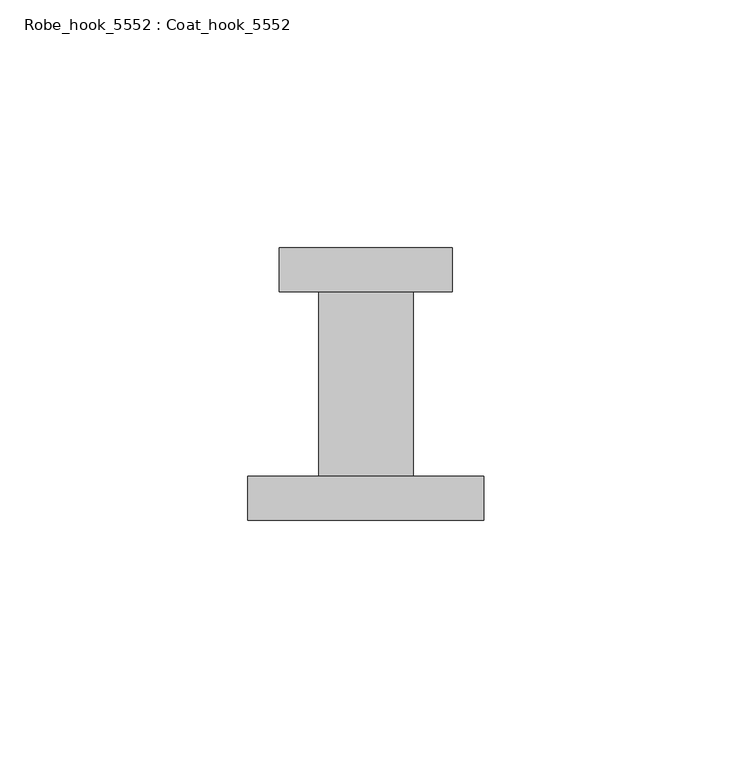
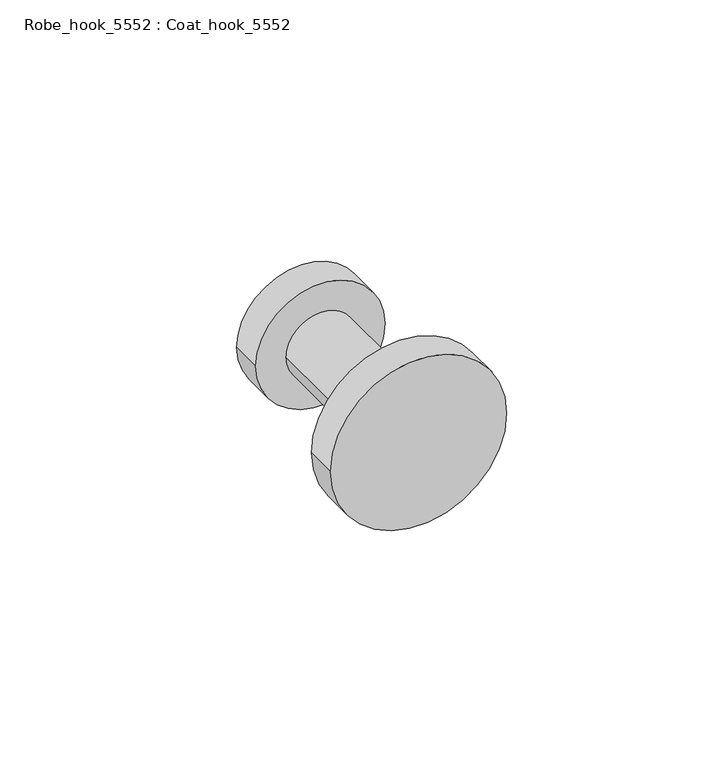
"""IFC4 building model written with IfcOpenShell, lengths in millimetres: proxy geometry, Robe_hook_5552 : Coat_hook_5552."""

from ifc_helpers import new_model, si_unit, point, frame, frame_2d, origin, place, context, project, spatial, circle_curve, trimmed, segment, composite_curve, outline, extrude, source, transform, mapped, element, save


def robe_hook_5552_coat_hook_5552_50ae73f2(model_context):
    return source(origin(), model_context, "Body", "SweptSolid", [
        extrude(outline(composite_curve([segment(trimmed(circle_curve(frame_2d((1371.6, 0.0)), 17.4626016), [point((1371.6, 17.4626016))], [point((1371.6, -17.4626016))], False, "CARTESIAN"), True, "CONTINUOUS"), segment(trimmed(circle_curve(frame_2d((1371.6, 0.0)), 17.4626016), [point((1371.6, -17.4626016))], [point((1371.6, 17.4626016))], False, "CARTESIAN"), True, "CONTINUOUS")], self_intersect=False)), frame((0.0, 46.0399015, 0.0), z_axis=(0.0, 1.0, 0.0), x_axis=(0.0, 0.0, 1.0)), (0.0, 0.0, 1.0), 8.9023917),
        extrude(outline(composite_curve([segment(trimmed(circle_curve(frame_2d((1371.6, 0.0)), 9.525), [point((1371.6, 9.525))], [point((1371.6, -9.525))], False, "CARTESIAN"), True, "CONTINUOUS"), segment(trimmed(circle_curve(frame_2d((1371.6, 0.0)), 9.525), [point((1371.6, -9.525))], [point((1371.6, 9.525))], False, "CARTESIAN"), True, "CONTINUOUS")], self_intersect=False)), frame((0.0, 8.9023917, 0.0), z_axis=(0.0, 1.0, 0.0), x_axis=(0.0, 0.0, 1.0)), (0.0, 0.0, 1.0), 37.1375098),
        extrude(outline(composite_curve([segment(trimmed(circle_curve(frame_2d((1371.6, 0.0)), 23.8125), [point((1371.6, 23.8125))], [point((1371.6, -23.8125))], False, "CARTESIAN"), True, "CONTINUOUS"), segment(trimmed(circle_curve(frame_2d((1371.6, 0.0)), 23.8125), [point((1371.6, -23.8125))], [point((1371.6, 23.8125))], False, "CARTESIAN"), True, "CONTINUOUS")], self_intersect=False)), frame((0.0, 0.0, 0.0), z_axis=(0.0, 1.0, 0.0), x_axis=(0.0, 0.0, 1.0)), (0.0, 0.0, 1.0), 8.9023917),
    ])


if __name__ == "__main__":
    model = new_model("IFC4")
    model_context = context("Model", 3, world=origin())
    ifc_project = project(units=[si_unit("LENGTHUNIT", "METRE", prefix="MILLI")], contexts=[model_context])
    site = spatial("IfcSite", under=ifc_project)
    building = spatial("IfcBuilding", under=site)
    placement = place(None, origin())
    robe_hook_5552_coat_hook_5552_shape = robe_hook_5552_coat_hook_5552_50ae73f2(model_context)
    element("IfcBuildingElementProxy", 1, Name="Robe_hook_5552 : Coat_hook_5552", ObjectType="Robe_hook_5552 : Coat_hook_5552", at=placement, inside=building, context=model_context, shape_type="MappedRepresentation", body=[
        mapped(robe_hook_5552_coat_hook_5552_shape, transform((0.0, 0.0, 0.0), x_axis=(1.0, 0.0, 0.0), y_axis=(0.0, 1.0, 0.0), z_axis=(0.0, 0.0, 1.0))),
    ])
    save(model, "model.ifc")

# Revit data of these elements
# Type "Robe_hook_5552 : Coat_hook_5552"
#   Keynote = "M10281600.03"
